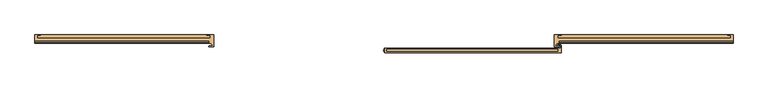
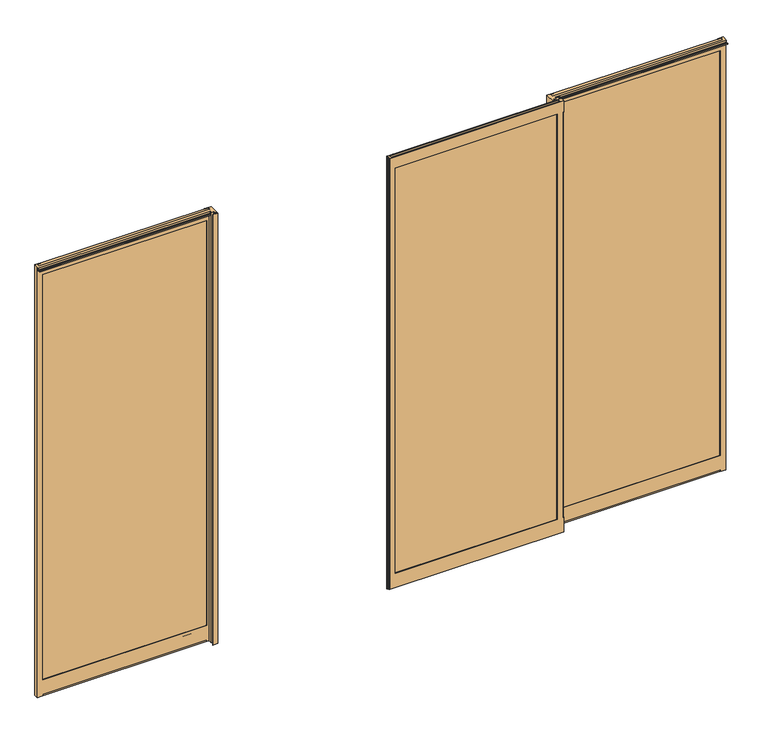
"""IFC4 building model written with IfcOpenShell, lengths in millimetres: door geometry, Otomatik Kapı-Tek Kanat : Otomatik Kapı - Tek Kanat."""

from ifc_helpers import new_model, si_unit, point, frame, frame_2d, origin, place, context, project, spatial, polyline, circle_curve, trimmed, segment, composite_curve, outline, extrude, source, transform, mapped, element, save
from ifc_brep_helpers import plane_surface, cylinder_surface, revolved_surface, advanced_brep


def door_bd07e04d(model_context):
    return source(origin(), model_context, "Body", "SolidModel", [
        advanced_brep(
        [(1555.0015, -107.5, 0.0), (1580.0, -107.5, 0.0), (1580.0, -127.5, 0.0), (1555.0015331, -127.5, 0.0), (1555.0015331, -125.4999765, 0.0), (801.3014669, -125.4999173, 0.0), (801.3014669, -127.5, 0.0), (791.2999735, -127.5, 0.0), (791.2999735, -145.3999231, 0.0), (781.2999977, -145.3999231, 0.0), (781.2999977, -148.5928431, 0.0), (776.0928913, -153.7999496, 0.0), (773.3, -153.7999496, 0.0), (773.3, -156.8999681, 0.0), (790.3010861, -156.8999681, 0.0), (794.3010782, -159.2093663, 0.0), (794.3010782, -160.4999631, 0.0), (771.3, -160.4999631, 0.0), (771.3, -107.5, 0.0), (801.3015, -107.5, 0.0), (801.3015, -109.5000196, 0.0), (1555.0015, -109.4993325, 0.0), (1555.0015331, -127.4999986, 8.0), (1555.0015331, -125.4999737, 8.0), (1555.0015331, -125.499275, 2045.5000009), (1555.0015331, -125.4999497, 77.9996358), (1555.0015331, -127.4999861, 77.9996641), (1555.0015331, -127.4996356, 2045.5000009), (1570.0015, -109.4992492, 62.9982401), (1570.0015, -125.499955, 62.9982401), (1570.0015, -125.499275, 2060.5013187), (1570.0015, -109.4966078, 2060.5013187), (1570.0015, -109.4993325, 2091.0), (1570.0015, -109.4993325, 2089.5000015), (1570.0015, -120.9996409, 2089.5000015), (1570.0015, -122.4996398, 2091.0003428), (1555.0015, -109.4993325, 8.0), (1555.0015, -107.4999999, 8.0), (1555.0015, -107.5, 2091.0), (1555.0015, -107.4999825, 2089.5000015), (1555.0015, -109.4993325, 2089.5000015), (1555.0015, -109.4993325, 2091.0), (1555.0015, -107.4999825, 2045.500003), (1555.0015, -107.4999993, 77.9999376), (1555.0015, -109.4992286, 77.9999379), (1555.0015, -109.4966078, 2045.500003), (801.3015, -107.4999999, 8.0), (801.3015, -109.5000063, 8.0), (801.3015, -109.5000196, 2091.0), (801.3015, -109.5000196, 2089.5000015), (801.3015, -107.4999825, 2089.5000015), (801.3015, -107.5, 2091.0), (801.3015, -109.4966078, 2045.500003), (801.3015, -109.4998895, 77.9999379), (801.3015, -107.4999993, 77.9999376), (801.3015, -107.4999825, 2045.500003), (786.3, -125.4998977, 62.9982401), (786.3, -109.4999153, 62.9982401), (786.3, -109.4966078, 2060.5013187), (786.3, -125.499275, 2060.5013187), (786.3, -122.4996398, 2091.0003428), (786.3, -120.9996409, 2089.5000015), (786.3, -109.5000196, 2089.5000015), (786.3, -109.5000196, 2091.0), (801.3014669, -125.5003878, 8.0), (801.3014669, -127.4999986, 8.0), (801.3014669, -127.4996356, 2045.5000009), (801.3014669, -127.4999861, 77.9996641), (801.3014669, -125.4998928, 77.9996358), (801.3014669, -125.499275, 2045.5000009), (791.2999735, -127.4996356, 2088.5000006), (791.2999735, -131.9000049, 2088.5000006), (791.2999735, -131.9000049, 2081.0024373), (791.2999735, -135.4001347, 2077.4999998), (791.2999735, -145.0000043, 2077.4999987), (791.2999735, -145.0000043, 2082.9999987), (791.2999735, -143.0000044, 2082.9999987), (791.2999735, -143.0000044, 2079.9999989), (791.2999735, -135.4000924, 2079.9999989), (791.2999735, -134.3999191, 2081.0001307), (791.2999735, -134.3999191, 2091.0003428), (791.2999735, -145.3999231, 2091.0), (781.2999977, -145.3999231, 2091.0), (771.3, -160.4999631, 2091.0), (794.3010782, -160.4999631, 2091.0), (1580.0, -107.5, 2091.0), (1580.0, -134.3999191, 2091.0003428), (1580.0, -134.3999191, 2081.0001307), (1580.0, -135.4000924, 2079.9999572), (1580.0, -143.0000044, 2079.9999989), (1580.0, -143.0000044, 2082.9999987), (1580.0, -145.0000043, 2082.9999987), (1580.0, -145.0000043, 2077.4999987), (1580.0, -135.4001347, 2077.4999987), (1580.0, -131.9000049, 2081.0024373), (1580.0, -131.9000049, 2088.5000006), (1580.0, -127.4996356, 2088.5000006), (771.3, -107.5, 2091.0), (794.3010782, -159.2093663, 2091.0003428), (790.3010861, -156.8999681, 2091.0003428), (773.3, -156.8999681, 2091.0003428), (773.3, -153.7999496, 2091.0003428), (776.0928913, -153.7999496, 2091.0003428), (781.2999977, -148.5928431, 2091.0003428)],
        [
            (0, 1),
            (1, 2),
            (2, 3),
            (3, 4),
            (4, 5),
            (5, 6),
            (6, 7),
            (7, 8),
            (8, 9),
            (9, 10),
            (10, 11),
            (11, 12),
            (12, 13),
            (13, 14),
            (14, 15),
            (15, 16),
            (16, 17),
            (17, 18),
            (18, 19),
            (19, 20),
            (20, 21),
            (21, 0),
            (3, 22),
            (22, 23),
            (23, 4),
            (24, 25),
            (25, 26),
            (26, 27),
            (27, 24),
            (28, 29),
            (29, 30),
            (30, 31),
            (31, 28),
            (32, 33),
            (33, 34),
            (34, 35),
            (35, 32),
            (21, 36),
            (36, 37),
            (37, 0),
            (38, 39),
            (39, 40),
            (40, 41),
            (41, 38),
            (42, 43),
            (43, 44),
            (44, 45),
            (45, 42),
            (19, 46),
            (46, 47),
            (47, 20),
            (48, 49),
            (49, 50),
            (50, 51),
            (51, 48),
            (52, 53),
            (53, 54),
            (54, 55),
            (55, 52),
            (56, 57),
            (57, 58),
            (58, 59),
            (59, 56),
            (60, 61),
            (61, 62),
            (62, 63),
            (63, 60),
            (5, 64),
            (64, 65),
            (65, 6),
            (66, 67),
            (67, 68),
            (68, 69),
            (69, 66),
            (70, 71),
            (71, 72),
            (72, 73, circle_curve(frame((791.2999735, -135.4001351, 2081.0001307), z_axis=(-1.0, 0.0, 0.0), x_axis=(0.0, 0.0, 1.0)), 3.5001309)),
            (73, 74),
            (74, 75),
            (75, 76),
            (76, 77),
            (77, 78),
            (78, 79, circle_curve(frame((791.2999735, -135.4000925, 2081.0001307), z_axis=(1.0, 0.0, 0.0), x_axis=(0.0, 0.0, 1.0)), 1.0001735)),
            (79, 80),
            (80, 81),
            (81, 8),
            (7, 70),
            (82, 9),
            (81, 82),
            (83, 17),
            (16, 84),
            (84, 83),
            (45, 52),
            (55, 42),
            (30, 59),
            (58, 31),
            (27, 66),
            (69, 24),
            (25, 68),
            (67, 26),
            (56, 29),
            (28, 57),
            (43, 54),
            (53, 44),
            (1, 85),
            (85, 86),
            (86, 87),
            (87, 88, circle_curve(frame((1580.0, -135.4000925, 2081.0001307), z_axis=(-1.0, 0.0, 0.0), x_axis=(0.0, 0.0, 1.0)), 1.0001735)),
            (88, 89),
            (89, 90),
            (90, 91),
            (91, 92),
            (92, 93),
            (93, 94, circle_curve(frame((1580.0, -135.4001351, 2081.0001307), z_axis=(1.0, 0.0, 0.0), x_axis=(0.0, 0.0, 1.0)), 3.5001309)),
            (94, 95),
            (95, 96),
            (96, 2),
            (83, 97),
            (97, 18),
            (41, 32),
            (35, 60),
            (63, 48),
            (51, 97),
            (84, 98),
            (98, 99),
            (99, 100),
            (100, 101),
            (101, 102),
            (102, 103),
            (103, 82),
            (80, 86),
            (85, 38),
            (37, 46),
            (50, 39),
            (40, 33),
            (62, 49),
            (96, 70),
            (65, 22),
            (34, 61),
            (95, 71),
            (94, 72),
            (93, 73),
            (92, 74),
            (91, 75),
            (90, 76),
            (89, 77),
            (88, 78),
            (87, 79),
            (103, 10),
            (102, 11),
            (101, 12),
            (100, 13),
            (99, 14),
            (98, 15),
            (36, 47),
            (23, 64),
        ],
        [
            plane_surface(frame((1580.0, -107.5, 0.0), z_axis=(0.0, 0.0, -1.0), x_axis=(0.0, -1.0, 0.0))),
            plane_surface(frame((1555.0015331, -127.5, 2091.0), z_axis=(-1.0, 0.0, 0.0), x_axis=(0.0, 0.0, -1.0))),
            plane_surface(frame((1570.0015, -125.4999765, 2091.0), z_axis=(-1.0, 0.0, 0.0), x_axis=(0.0, 0.0, -1.0))),
            plane_surface(frame((1555.0015, -109.4993325, 2091.0), z_axis=(-1.0, 0.0, 0.0), x_axis=(0.0, 0.0, -1.0))),
            plane_surface(frame((801.3015, -107.5, 2091.0), z_axis=(1.0, 0.0, 0.0), x_axis=(0.0, 0.0, -1.0))),
            plane_surface(frame((786.3, -109.5000196, 2091.0), z_axis=(1.0, 0.0, 0.0), x_axis=(0.0, 0.0, -1.0))),
            plane_surface(frame((801.3014669, -125.4999173, 2091.0), z_axis=(1.0, 0.0, 0.0), x_axis=(0.0, 0.0, -1.0))),
            plane_surface(frame((791.2999735, -127.5, 2091.0), z_axis=(1.0, 0.0, 0.0), x_axis=(0.0, 0.0, -1.0))),
            plane_surface(frame((791.2999735, -145.3999231, 2091.0), z_axis=(0.0, -1.0, 0.0), x_axis=(0.0, 0.0, -1.0))),
            plane_surface(frame((794.3010782, -160.4999631, 2091.0), z_axis=(0.0, -1.0, 0.0), x_axis=(0.0, 0.0, -1.0))),
            plane_surface(frame((1580.0, -107.4999825, 2045.500003), z_axis=(0.0, 0.0, -1.0), x_axis=(-1.0, 0.0, 0.0))),
            plane_surface(frame((1580.0, -109.4966078, 2060.5013187), z_axis=(0.0, 0.0, -1.0), x_axis=(-1.0, 0.0, 0.0))),
            plane_surface(frame((1580.0, -125.499275, 2045.5000009), z_axis=(0.0, 0.0, -1.0), x_axis=(-1.0, 0.0, 0.0))),
            plane_surface(frame((1580.0, -127.5, 77.9996641), z_axis=(0.0, 1.4132729652639372e-05, 0.999999999900133), x_axis=(-1.0, 0.0, 0.0))),
            plane_surface(frame((1580.0, -125.4999765, 62.9982401), z_axis=(0.0, 0.0, 1.0), x_axis=(-1.0, 0.0, 0.0))),
            plane_surface(frame((1580.0, -109.4999015, 77.9999379), z_axis=(0.0, 1.674987849023181e-07, 0.999999999999986), x_axis=(-1.0, 0.0, 0.0))),
            plane_surface(frame((1580.0, -107.5, 2091.0), z_axis=(1.0, 0.0, 0.0), x_axis=(0.0, -1.0, 0.0))),
            plane_surface(frame((771.3, -107.5, 2091.0), z_axis=(-1.0, 0.0, 0.0), x_axis=(0.0, -1.0, 0.0))),
            plane_surface(frame((1580.0, -134.3999191, 2091.0003428), z_axis=(0.0, 0.0, 1.0), x_axis=(-1.0, 0.0, 0.0))),
            plane_surface(frame((1580.0, -107.4999825, 2089.5000015), z_axis=(0.0, 1.0, 0.0), x_axis=(-1.0, 0.0, 0.0))),
            plane_surface(frame((1580.0, -109.4966078, 2045.500003), z_axis=(0.0, -1.0, 0.0), x_axis=(-1.0, 0.0, 0.0))),
            plane_surface(frame((1580.0, -125.499275, 2060.5013187), z_axis=(0.0, 1.0, 0.0), x_axis=(-1.0, 0.0, 0.0))),
            plane_surface(frame((1580.0, -127.4996356, 2045.5000009), z_axis=(0.0, -1.0, 0.0), x_axis=(-1.0, 0.0, 0.0))),
            plane_surface(frame((1580.0, -122.4996398, 2091.0003428), z_axis=(0.0, 0.7071874732725993, 0.7070260798911995), x_axis=(-1.0, 0.0, 0.0))),
            plane_surface(frame((1580.0, -120.9996409, 2089.5000015), z_axis=(0.0, 0.0, 1.0), x_axis=(-1.0, 0.0, 0.0))),
            plane_surface(frame((1580.0, -127.4996356, 2088.5000006), z_axis=(0.0, 0.0, -1.0), x_axis=(-1.0, 0.0, 0.0))),
            plane_surface(frame((1580.0, -131.9000049, 2088.5000006), z_axis=(0.0, 1.0, 0.0), x_axis=(-1.0, 0.0, 0.0))),
            cylinder_surface(frame((1580.0, -135.4001351, 2081.0001307), z_axis=(1.0, 0.0, 0.0), x_axis=(0.0, 0.0, 1.0)), 3.5001309),
            plane_surface(frame((1580.0, -135.4001347, 2077.4999987), z_axis=(0.0, 0.0, -1.0), x_axis=(-1.0, 0.0, 0.0))),
            plane_surface(frame((1580.0, -145.0000043, 2077.4999987), z_axis=(0.0, -1.0, 0.0), x_axis=(-1.0, 0.0, 0.0))),
            plane_surface(frame((1580.0, -145.0000043, 2082.9999987), z_axis=(0.0, 0.0, 1.0), x_axis=(-1.0, 0.0, 0.0))),
            plane_surface(frame((1580.0, -143.0000044, 2082.9999987), z_axis=(0.0, 1.0, 0.0), x_axis=(-1.0, 0.0, 0.0))),
            plane_surface(frame((1580.0, -143.0000044, 2079.9999989), z_axis=(0.0, 0.0, 1.0), x_axis=(-1.0, 0.0, 0.0))),
            revolved_surface(polyline([(791.2999735, -135.4000925, 2082.0003042000003), (1580.0, -135.4000925, 2082.0003042000003)]), (1580.0, -135.4000925, 2081.0001307), (-1.0, 0.0, 0.0)),
            plane_surface(frame((1580.0, -134.3999191, 2081.0001307), z_axis=(0.0, -1.0, 0.0), x_axis=(-1.0, 0.0, 0.0))),
            plane_surface(frame((781.2999977, -145.3999231, 2091.0), z_axis=(1.0, 0.0, 0.0), x_axis=(0.0, 0.0, -1.0))),
            plane_surface(frame((781.2999977, -148.5928431, 2091.0), z_axis=(0.7071067811865539, -0.7071067811865412, 0.0), x_axis=(0.0, 0.0, -1.0))),
            plane_surface(frame((776.0928913, -153.7999496, 2091.0), z_axis=(0.0, -1.0, 0.0), x_axis=(0.0, 0.0, -1.0))),
            plane_surface(frame((773.3, -153.7999496, 2091.0), z_axis=(1.0, 0.0, 0.0), x_axis=(0.0, 0.0, -1.0))),
            plane_surface(frame((773.3, -156.8999681, 2091.0), z_axis=(0.0, 1.0, 0.0), x_axis=(0.0, 0.0, -1.0))),
            plane_surface(frame((790.3010861, -156.8999681, 2091.0), z_axis=(0.5000002758229711, 0.8660252445379135, 0.0), x_axis=(0.0, 0.0, -1.0))),
            plane_surface(frame((794.3010782, -159.2093663, 2091.0), z_axis=(1.0, 0.0, 0.0), x_axis=(0.0, 0.0, -1.0))),
            plane_surface(frame((1580.0, -107.5000072, 8.0), z_axis=(0.0, 0.0, -1.0), x_axis=(-1.0, 0.0, 0.0))),
            plane_surface(frame((1580.0, -109.4993325, 8.0), z_axis=(0.0, 1.0, 0.0), x_axis=(-1.0, 0.0, 0.0))),
            plane_surface(frame((1580.0, -125.5003878, 0.0), z_axis=(0.0, -1.0, 0.0), x_axis=(-1.0, 0.0, 0.0))),
            plane_surface(frame((1580.0, -125.5003878, 8.0), z_axis=(0.0, 0.0, -1.0), x_axis=(-1.0, 0.0, 0.0))),
        ],
        [
            (0, [[1, 2, 3, 4, 5, 6, 7, 8, 9, 10, 11, 12, 13, 14, 15, 16, 17, 18, 19, 20, 21, 22]]),
            (1, [[23, 24, 25, -4]]),
            (1, [[26, 27, 28, 29]]),
            (2, [[30, 31, 32, 33]]),
            (2, [[34, 35, 36, 37]]),
            (3, [[38, 39, 40, -22]]),
            (3, [[41, 42, 43, 44]]),
            (3, [[45, 46, 47, 48]]),
            (4, [[49, 50, 51, -20]]),
            (4, [[52, 53, 54, 55]]),
            (4, [[56, 57, 58, 59]]),
            (5, [[60, 61, 62, 63]]),
            (5, [[64, 65, 66, 67]]),
            (6, [[68, 69, 70, -6]]),
            (6, [[71, 72, 73, 74]]),
            (7, [[75, 76, 77, 78, 79, 80, 81, 82, 83, 84, 85, 86, -8, 87]]),
            (8, [[88, -9, -86, 89]]),
            (9, [[90, -17, 91, 92]]),
            (10, [[93, -59, 94, -48]]),
            (11, [[95, -62, 96, -32]]),
            (12, [[97, -74, 98, -29]]),
            (13, [[-27, 99, -72, 100]]),
            (14, [[-60, 101, -30, 102]]),
            (15, [[-46, 103, -57, 104]]),
            (16, [[105, 106, 107, 108, 109, 110, 111, 112, 113, 114, 115, 116, 117, -2]]),
            (17, [[118, 119, -18, -90]]),
            (18, [[-44, 120, -37, 121, -67, 122, -55, 123, -118, -92, 124, 125, 126, 127, 128, 129, 130, -89, -85, 131, -106, 132]]),
            (19, [[-105, -1, -40, 133, -49, -19, -119, -123, -54, 134, -41, -132], [-94, -58, -103, -45]]),
            (20, [[-43, 135, -34, -120]]),
            (20, [[-66, 136, -52, -122]]),
            (20, [[-61, -102, -33, -96], [-47, -104, -56, -93]]),
            (21, [[-31, -101, -63, -95], [-73, -99, -26, -98]]),
            (22, [[-117, 137, -87, -7, -70, 138, -23, -3], [-97, -28, -100, -71]]),
            (23, [[139, -64, -121, -36]]),
            (24, [[-135, -42, -134, -53, -136, -65, -139, -35]]),
            (25, [[140, -75, -137, -116]]),
            (26, [[141, -76, -140, -115]]),
            (27, [[142, -77, -141, -114]]),
            (28, [[143, -78, -142, -113]]),
            (29, [[144, -79, -143, -112]]),
            (30, [[145, -80, -144, -111]]),
            (31, [[146, -81, -145, -110]]),
            (32, [[147, -82, -146, -109]]),
            (33, [[148, -83, -147, -108]]),
            (34, [[-131, -84, -148, -107]]),
            (35, [[149, -10, -88, -130]]),
            (36, [[150, -11, -149, -129]]),
            (37, [[151, -12, -150, -128]]),
            (38, [[152, -13, -151, -127]]),
            (39, [[153, -14, -152, -126]]),
            (40, [[154, -15, -153, -125]]),
            (41, [[-91, -16, -154, -124]]),
            (42, [[-50, -133, -39, 155]]),
            (43, [[-51, -155, -38, -21]]),
            (44, [[-25, 156, -68, -5]]),
            (45, [[-69, -156, -24, -138]]),
        ],
    ),
        extrude(outline(polyline([(788.792088, -114.5000025), (1567.9612743, -114.5000025), (1567.9612743, -124.5000025), (788.792088, -124.5000025), (788.792088, -114.5000025)])), frame((0.0, 0.0, 70.0), z_axis=(0.0, 0.0, 1.0), x_axis=(1.0, 0.0, 0.0)), (0.0, 0.0, 1.0), 1989.0),
        advanced_brep(
        [(-1555.0015, -107.5, 0.0), (-1555.0015, -109.4993325, 0.0), (-801.3015, -109.4966078, 0.0), (-801.3015, -107.5, 0.0), (-771.3, -107.5, 0.0), (-771.3, -160.4999631, 0.0), (-794.3010782, -160.4999631, 0.0), (-794.3010782, -159.2093663, 0.0), (-790.3010861, -156.8999681, 0.0), (-773.3, -156.8999681, 0.0), (-773.3, -153.7999496, 0.0), (-776.0928913, -153.7999496, 0.0), (-781.2999977, -148.5928431, 0.0), (-781.2999977, -145.3999231, 0.0), (-791.2999735, -145.3999231, 0.0), (-791.2999735, -127.5, 0.0), (-801.3014669, -127.5, 0.0), (-801.3014669, -125.4999173, 0.0), (-1555.0015331, -125.499275, 0.0), (-1555.0015331, -127.5, 0.0), (-1580.0, -127.5, 0.0), (-1580.0, -107.5, 0.0), (-1555.0015331, -125.5003878, 8.0), (-1555.0015331, -127.4999986, 8.0), (-1555.0015331, -125.499275, 2045.5000009), (-1555.0015331, -127.4996356, 2045.5000009), (-1555.0015331, -127.4999861, 77.9996641), (-1555.0015331, -125.4999497, 77.9996358), (-1570.0015, -109.4993325, 2091.0), (-1570.0015, -122.4996398, 2091.0003428), (-1570.0015, -120.9996409, 2089.5000015), (-1570.0015, -109.4993325, 2089.5000015), (-1570.0015, -109.4992492, 62.9982401), (-1570.0015, -109.4966078, 2060.5013187), (-1570.0015, -125.499275, 2060.5013187), (-1570.0015, -125.499955, 62.9982401), (-1555.0015, -107.4999999, 8.0), (-1555.0015, -109.4993218, 8.0), (-1555.0015, -107.4999825, 2045.500003), (-1555.0015, -109.4966078, 2045.500003), (-1555.0015, -109.4992286, 77.9999379), (-1555.0015, -107.4999993, 77.9999376), (-1555.0015, -107.5, 2091.0), (-1555.0015, -109.4993325, 2091.0), (-1555.0015, -109.4993325, 2089.5000015), (-1555.0015, -107.4999825, 2089.5000015), (-801.3015, -109.4993325, 8.0), (-801.3015, -107.4999999, 8.0), (-801.3015, -109.4966078, 2045.500003), (-801.3015, -107.4999825, 2045.500003), (-801.3015, -107.4999993, 77.9999376), (-801.3015, -109.4998895, 77.9999379), (-801.3015, -109.5000196, 2091.0), (-801.3015, -107.5, 2091.0), (-801.3015, -107.4999825, 2089.5000015), (-801.3015, -109.5000196, 2089.5000015), (-786.3, -122.4996398, 2091.0003428), (-786.3, -109.5000196, 2091.0), (-786.3, -109.5000196, 2089.5000015), (-786.3, -120.9996409, 2089.5000015), (-786.3, -125.4998977, 62.9982401), (-786.3, -125.499275, 2060.5013187), (-786.3, -109.4966078, 2060.5013187), (-786.3, -109.4999153, 62.9982401), (-801.3014669, -127.4999986, 8.0), (-801.3014669, -125.4999148, 8.0), (-801.3014669, -127.4996356, 2045.5000009), (-801.3014669, -125.499275, 2045.5000009), (-801.3014669, -125.4998928, 77.9996358), (-801.3014669, -127.4999861, 77.9996641), (-791.2999735, -127.4996356, 2088.5000006), (-791.2999735, -145.3999231, 2091.0), (-791.2999735, -134.3999191, 2091.0003428), (-791.2999735, -134.3999191, 2081.0001307), (-791.2999735, -135.4000924, 2079.9999572), (-791.2999735, -143.0000043, 2079.9999989), (-791.2999735, -143.0000043, 2082.9999987), (-791.2999735, -145.0000043, 2082.9999987), (-791.2999735, -145.0000043, 2077.4999987), (-791.2999735, -135.4001347, 2077.4999987), (-791.2999735, -131.9000049, 2081.0024373), (-791.2999735, -131.9000049, 2088.5000006), (-781.2999977, -145.3999231, 2091.0), (-771.3, -160.4999631, 2091.0), (-794.3010782, -160.4999631, 2091.0), (-1580.0, -127.4996356, 2088.5000006), (-1580.0, -131.9000049, 2088.5000006), (-1580.0, -131.9000049, 2081.0024373), (-1580.0, -135.4001347, 2077.4999998), (-1580.0, -145.0000043, 2077.4999987), (-1580.0, -145.0000043, 2082.9999987), (-1580.0, -143.0000043, 2082.9999987), (-1580.0, -143.0000043, 2079.9999989), (-1580.0, -135.400135, 2079.9999989), (-1580.0, -134.3999191, 2081.0001307), (-1580.0, -134.3999191, 2091.0003428), (-1580.0, -107.5, 2091.0), (-771.3, -107.5, 2091.0), (-781.2999977, -148.5928431, 2091.0003428), (-776.0928913, -153.7999496, 2091.0003428), (-773.3, -153.7999496, 2091.0003428), (-773.3, -156.8999681, 2091.0003428), (-790.3010861, -156.8999681, 2091.0003428), (-794.3010782, -159.2093663, 2091.0003428)],
        [
            (0, 1),
            (1, 2),
            (2, 3),
            (3, 4),
            (4, 5),
            (5, 6),
            (6, 7),
            (7, 8),
            (8, 9),
            (9, 10),
            (10, 11),
            (11, 12),
            (12, 13),
            (13, 14),
            (14, 15),
            (15, 16),
            (16, 17),
            (17, 18),
            (18, 19),
            (19, 20),
            (20, 21),
            (21, 0),
            (18, 22),
            (22, 23),
            (23, 19),
            (24, 25),
            (25, 26),
            (26, 27),
            (27, 24),
            (28, 29),
            (29, 30),
            (30, 31),
            (31, 28),
            (32, 33),
            (33, 34),
            (34, 35),
            (35, 32),
            (0, 36),
            (36, 37),
            (37, 1),
            (38, 39),
            (39, 40),
            (40, 41),
            (41, 38),
            (42, 43),
            (43, 44),
            (44, 45),
            (45, 42),
            (2, 46),
            (46, 47),
            (47, 3),
            (48, 49),
            (49, 50),
            (50, 51),
            (51, 48),
            (52, 53),
            (53, 54),
            (54, 55),
            (55, 52),
            (56, 57),
            (57, 58),
            (58, 59),
            (59, 56),
            (60, 61),
            (61, 62),
            (62, 63),
            (63, 60),
            (16, 64),
            (64, 65),
            (65, 17),
            (66, 67),
            (67, 68),
            (68, 69),
            (69, 66),
            (70, 15),
            (14, 71),
            (71, 72),
            (72, 73),
            (73, 74, circle_curve(frame((-791.2999735, -135.4000925, 2081.0001307), z_axis=(-1.0, 0.0, 0.0), x_axis=(0.0, 0.0, 1.0)), 1.0001735)),
            (74, 75),
            (75, 76),
            (76, 77),
            (77, 78),
            (78, 79),
            (79, 80, circle_curve(frame((-791.2999735, -135.4001351, 2081.0001307), z_axis=(1.0, 0.0, 0.0), x_axis=(0.0, 0.0, 1.0)), 3.5001309)),
            (80, 81),
            (81, 70),
            (82, 71),
            (13, 82),
            (83, 84),
            (84, 6),
            (5, 83),
            (38, 49),
            (48, 39),
            (33, 62),
            (61, 34),
            (24, 67),
            (66, 25),
            (26, 69),
            (68, 27),
            (63, 32),
            (35, 60),
            (40, 51),
            (50, 41),
            (20, 85),
            (85, 86),
            (86, 87),
            (87, 88, circle_curve(frame((-1580.0, -135.4001351, 2081.0001307), z_axis=(-1.0, 0.0, 0.0), x_axis=(0.0, 0.0, 1.0)), 3.5001309)),
            (88, 89),
            (89, 90),
            (90, 91),
            (91, 92),
            (92, 93),
            (93, 94, circle_curve(frame((-1580.0, -135.4000925, 2081.0001307), z_axis=(1.0, 0.0, 0.0), x_axis=(0.0, 0.0, 1.0)), 1.0001735)),
            (94, 95),
            (95, 96),
            (96, 21),
            (4, 97),
            (97, 83),
            (42, 96),
            (95, 72),
            (82, 98),
            (98, 99),
            (99, 100),
            (100, 101),
            (101, 102),
            (102, 103),
            (103, 84),
            (97, 53),
            (52, 57),
            (56, 29),
            (28, 43),
            (45, 54),
            (47, 36),
            (55, 58),
            (31, 44),
            (23, 64),
            (70, 85),
            (59, 30),
            (81, 86),
            (80, 87),
            (79, 88),
            (78, 89),
            (77, 90),
            (76, 91),
            (75, 92),
            (74, 93),
            (73, 94),
            (12, 98),
            (11, 99),
            (10, 100),
            (9, 101),
            (8, 102),
            (7, 103),
            (46, 37),
            (65, 22),
        ],
        [
            plane_surface(frame((-1580.0, -107.5, 0.0), z_axis=(0.0, 0.0, -1.0), x_axis=(0.0, -1.0, 0.0))),
            plane_surface(frame((-1555.0015331, -127.5, 2091.0), z_axis=(1.0, 0.0, 0.0), x_axis=(0.0, 0.0, -1.0))),
            plane_surface(frame((-1570.0015, -125.4999765, 2091.0), z_axis=(1.0, 0.0, 0.0), x_axis=(0.0, 0.0, -1.0))),
            plane_surface(frame((-1555.0015, -109.4993325, 2091.0), z_axis=(1.0, 0.0, 0.0), x_axis=(0.0, 0.0, -1.0))),
            plane_surface(frame((-801.3015, -107.5, 2091.0), z_axis=(-1.0, 0.0, 0.0), x_axis=(0.0, 0.0, -1.0))),
            plane_surface(frame((-786.3, -109.5000196, 2091.0), z_axis=(-1.0, 0.0, 0.0), x_axis=(0.0, 0.0, -1.0))),
            plane_surface(frame((-801.3014669, -125.4999173, 2091.0), z_axis=(-1.0, 0.0, 0.0), x_axis=(0.0, 0.0, -1.0))),
            plane_surface(frame((-791.2999735, -127.5, 2091.0), z_axis=(-1.0, 0.0, 0.0), x_axis=(0.0, 0.0, -1.0))),
            plane_surface(frame((-791.2999735, -145.3999231, 2091.0), z_axis=(0.0, -1.0, 0.0), x_axis=(0.0, 0.0, -1.0))),
            plane_surface(frame((-794.3010782, -160.4999631, 2091.0), z_axis=(0.0, -1.0, 0.0), x_axis=(0.0, 0.0, -1.0))),
            plane_surface(frame((-1580.0, -107.4999825, 2045.500003), z_axis=(0.0, 0.0, -1.0), x_axis=(1.0, 0.0, 0.0))),
            plane_surface(frame((-1580.0, -109.4966078, 2060.5013187), z_axis=(0.0, 0.0, -1.0), x_axis=(1.0, 0.0, 0.0))),
            plane_surface(frame((-1580.0, -125.499275, 2045.5000009), z_axis=(0.0, 0.0, -1.0), x_axis=(1.0, 0.0, 0.0))),
            plane_surface(frame((-1580.0, -127.5, 77.9996641), z_axis=(0.0, 1.4132729652639372e-05, 0.999999999900133), x_axis=(1.0, 0.0, 0.0))),
            plane_surface(frame((-1580.0, -125.4999765, 62.9982401), z_axis=(0.0, 0.0, 1.0), x_axis=(1.0, 0.0, 0.0))),
            plane_surface(frame((-1580.0, -109.4999015, 77.9999379), z_axis=(0.0, 1.674987849023181e-07, 0.999999999999986), x_axis=(1.0, 0.0, 0.0))),
            plane_surface(frame((-1580.0, -107.5, 2091.0), z_axis=(-1.0, 0.0, 0.0), x_axis=(0.0, -1.0, 0.0))),
            plane_surface(frame((-771.3, -107.5, 2091.0), z_axis=(1.0, 0.0, 0.0), x_axis=(0.0, -1.0, 0.0))),
            plane_surface(frame((-1580.0, -134.3999191, 2091.0003428), z_axis=(0.0, 0.0, 1.0), x_axis=(1.0, 0.0, 0.0))),
            plane_surface(frame((-1580.0, -107.4999825, 2089.5000015), z_axis=(0.0, 1.0, 0.0), x_axis=(1.0, 0.0, 0.0))),
            plane_surface(frame((-1580.0, -109.4966078, 2045.500003), z_axis=(0.0, -1.0, 0.0), x_axis=(1.0, 0.0, 0.0))),
            plane_surface(frame((-1580.0, -125.499275, 2060.5013187), z_axis=(0.0, 1.0, 0.0), x_axis=(1.0, 0.0, 0.0))),
            plane_surface(frame((-1580.0, -127.4996356, 2045.5000009), z_axis=(0.0, -1.0, 0.0), x_axis=(1.0, 0.0, 0.0))),
            plane_surface(frame((-1580.0, -122.4996398, 2091.0003428), z_axis=(0.0, 0.7071874732725993, 0.7070260798911995), x_axis=(1.0, 0.0, 0.0))),
            plane_surface(frame((-1580.0, -120.9996409, 2089.5000015), z_axis=(0.0, 0.0, 1.0), x_axis=(1.0, 0.0, 0.0))),
            plane_surface(frame((-1580.0, -127.4996356, 2088.5000006), z_axis=(0.0, 0.0, -1.0), x_axis=(1.0, 0.0, 0.0))),
            plane_surface(frame((-1580.0, -131.9000049, 2088.5000006), z_axis=(0.0, 1.0, 0.0), x_axis=(1.0, 0.0, 0.0))),
            cylinder_surface(frame((-1580.0, -135.4001351, 2081.0001307), z_axis=(-1.0, 0.0, 0.0), x_axis=(0.0, 0.0, 1.0)), 3.5001309),
            plane_surface(frame((-1580.0, -135.4001347, 2077.4999987), z_axis=(0.0, 0.0, -1.0), x_axis=(1.0, 0.0, 0.0))),
            plane_surface(frame((-1580.0, -145.0000043, 2077.4999987), z_axis=(0.0, -1.0, 0.0), x_axis=(1.0, 0.0, 0.0))),
            plane_surface(frame((-1580.0, -145.0000043, 2082.9999987), z_axis=(0.0, 0.0, 1.0), x_axis=(1.0, 0.0, 0.0))),
            plane_surface(frame((-1580.0, -143.0000043, 2082.9999987), z_axis=(0.0, 1.0, 0.0), x_axis=(1.0, 0.0, 0.0))),
            plane_surface(frame((-1580.0, -143.0000043, 2079.9999989), z_axis=(0.0, 0.0, 1.0), x_axis=(1.0, 0.0, 0.0))),
            revolved_surface(polyline([(-791.2999735, -135.4000925, 2082.0003042000003), (-1580.0, -135.4000925, 2082.0003042000003)]), (-1580.0, -135.4000925, 2081.0001307), (1.0, 0.0, 0.0)),
            plane_surface(frame((-1580.0, -134.3999191, 2081.0001307), z_axis=(0.0, -1.0, 0.0), x_axis=(1.0, 0.0, 0.0))),
            plane_surface(frame((-781.2999977, -145.3999231, 2091.0), z_axis=(-1.0, 0.0, 0.0), x_axis=(0.0, 0.0, -1.0))),
            plane_surface(frame((-781.2999977, -148.5928431, 2091.0), z_axis=(-0.7071067811865539, -0.7071067811865412, 0.0), x_axis=(0.0, 0.0, -1.0))),
            plane_surface(frame((-776.0928913, -153.7999496, 2091.0), z_axis=(0.0, -1.0, 0.0), x_axis=(0.0, 0.0, -1.0))),
            plane_surface(frame((-773.3, -153.7999496, 2091.0), z_axis=(-1.0, 0.0, 0.0), x_axis=(0.0, 0.0, -1.0))),
            plane_surface(frame((-773.3, -156.8999681, 2091.0), z_axis=(0.0, 1.0, 0.0), x_axis=(0.0, 0.0, -1.0))),
            plane_surface(frame((-790.3010861, -156.8999681, 2091.0), z_axis=(-0.5000002758229711, 0.8660252445379135, 0.0), x_axis=(0.0, 0.0, -1.0))),
            plane_surface(frame((-794.3010782, -159.2093663, 2091.0), z_axis=(-1.0, 0.0, 0.0), x_axis=(0.0, 0.0, -1.0))),
            plane_surface(frame((-1580.0, -107.5000072, 8.0), z_axis=(0.0, 0.0, -1.0), x_axis=(1.0, 0.0, 0.0))),
            plane_surface(frame((-1580.0, -109.4993325, 8.0), z_axis=(0.0, 1.0, 0.0), x_axis=(1.0, 0.0, 0.0))),
            plane_surface(frame((-1580.0, -125.5003878, 0.0), z_axis=(0.0, -1.0, 0.0), x_axis=(1.0, 0.0, 0.0))),
            plane_surface(frame((-1580.0, -125.5003878, 8.0), z_axis=(0.0, 0.0, -1.0), x_axis=(1.0, 0.0, 0.0))),
        ],
        [
            (0, [[1, 2, 3, 4, 5, 6, 7, 8, 9, 10, 11, 12, 13, 14, 15, 16, 17, 18, 19, 20, 21, 22]]),
            (1, [[-19, 23, 24, 25]]),
            (1, [[26, 27, 28, 29]]),
            (2, [[30, 31, 32, 33]]),
            (2, [[34, 35, 36, 37]]),
            (3, [[-1, 38, 39, 40]]),
            (3, [[41, 42, 43, 44]]),
            (3, [[45, 46, 47, 48]]),
            (4, [[-3, 49, 50, 51]]),
            (4, [[52, 53, 54, 55]]),
            (4, [[56, 57, 58, 59]]),
            (5, [[60, 61, 62, 63]]),
            (5, [[64, 65, 66, 67]]),
            (6, [[-17, 68, 69, 70]]),
            (6, [[71, 72, 73, 74]]),
            (7, [[75, -15, 76, 77, 78, 79, 80, 81, 82, 83, 84, 85, 86, 87]]),
            (8, [[88, -76, -14, 89]]),
            (9, [[90, 91, -6, 92]]),
            (10, [[-41, 93, -52, 94]]),
            (11, [[-35, 95, -65, 96]]),
            (12, [[-26, 97, -71, 98]]),
            (13, [[99, -73, 100, -28]]),
            (14, [[101, -37, 102, -67]]),
            (15, [[103, -54, 104, -43]]),
            (16, [[-21, 105, 106, 107, 108, 109, 110, 111, 112, 113, 114, 115, 116, 117]]),
            (17, [[-92, -5, 118, 119]]),
            (18, [[120, -116, 121, -77, -88, 122, 123, 124, 125, 126, 127, 128, -90, -119, 129, -56, 130, -60, 131, -30, 132, -45]]),
            (19, [[-120, -48, 133, -57, -129, -118, -4, -51, 134, -38, -22, -117], [-44, -104, -53, -93]]),
            (20, [[-95, -34, -101, -66], [-94, -55, -103, -42]]),
            (20, [[-130, -59, 135, -61]]),
            (20, [[-132, -33, 136, -46]]),
            (21, [[-96, -64, -102, -36], [-97, -29, -100, -72]]),
            (22, [[-20, -25, 137, -68, -16, -75, 138, -105], [-74, -99, -27, -98]]),
            (23, [[-31, -131, -63, 139]]),
            (24, [[-32, -139, -62, -135, -58, -133, -47, -136]]),
            (25, [[-106, -138, -87, 140]]),
            (26, [[-107, -140, -86, 141]]),
            (27, [[-108, -141, -85, 142]]),
            (28, [[-109, -142, -84, 143]]),
            (29, [[-110, -143, -83, 144]]),
            (30, [[-111, -144, -82, 145]]),
            (31, [[-112, -145, -81, 146]]),
            (32, [[-113, -146, -80, 147]]),
            (33, [[-114, -147, -79, 148]]),
            (34, [[-115, -148, -78, -121]]),
            (35, [[-122, -89, -13, 149]]),
            (36, [[-123, -149, -12, 150]]),
            (37, [[-124, -150, -11, 151]]),
            (38, [[-125, -151, -10, 152]]),
            (39, [[-126, -152, -9, 153]]),
            (40, [[-127, -153, -8, 154]]),
            (41, [[-128, -154, -7, -91]]),
            (42, [[155, -39, -134, -50]]),
            (43, [[-2, -40, -155, -49]]),
            (44, [[-18, -70, 156, -23]]),
            (45, [[-137, -24, -156, -69]]),
        ],
    ),
        extrude(outline(polyline([(-788.792088, -114.5000025), (-788.792088, -124.5000025), (-1567.9612743, -124.5000025), (-1567.9612743, -114.5000025), (-788.792088, -114.5000025)])), frame((0.0, 0.0, 70.0), z_axis=(0.0, 0.0, 1.0), x_axis=(1.0, 0.0, 0.0)), (0.0, 0.0, 1.0), 1989.0),
        advanced_brep(
        [(802.5, -155.7669497, 8.0000212), (802.5, -187.3, 8.0000212), (2.5, -187.3, 8.0000212), (2.5, -167.3000082, 8.0000212), (800.5, -167.3, 8.0000212), (800.5, -155.8138546, 8.0000212), (799.4861454, -154.8, 8.0000212), (787.49925, -154.8, 8.0000212), (787.49925, -152.8, 8.0000212), (799.5330503, -152.8, 8.0000212), (787.49925, -180.7974169, 8.0000212), (787.49925, -173.8001834, 8.0000212), (12.4985, -173.8001834, 8.0000212), (12.4985, -180.7974169, 8.0000212), (800.5, -167.3, 2101.0), (2.5, -167.3, 2101.0), (2.5, -187.3, 2101.0), (802.5, -187.3, 2101.0), (802.5, -155.7669497, 2101.0), (799.5330503, -152.8, 2101.0), (787.49925, -152.8, 2101.0), (787.49925, -154.8, 2101.0), (799.4861454, -154.8, 2101.0), (800.5, -155.8138546, 2101.0), (787.49925, -172.299, 2101.0), (787.49925, -182.301, 2101.0), (12.4985, -182.301, 2101.0), (12.4985, -172.299, 2101.0), (802.5, -187.3, 2046.0007973), (802.5, -185.3, 2046.0007973), (802.5, -185.3, 2061.0007973), (802.5, -184.239458, 2061.0007973), (802.5, -184.239458, 62.9982446), (802.5, -185.3, 62.9982446), (802.5, -185.3, 78.000055), (802.5, -187.3, 78.000055), (772.4862373, -167.3, 2046.0004744), (772.4862373, -167.3, 77.9999799), (772.4862373, -169.2993721, 77.9999799), (772.4862373, -169.2993721, 2046.0004744), (787.49925, -169.2993721, 2061.0007973), (12.4985, -169.2993721, 2061.0007973), (12.4985, -169.2993721, 62.9982446), (787.49925, -169.2993721, 62.9982446), (27.4985, -169.2993721, 77.9999799), (27.4985, -169.2993721, 2046.0004744), (787.49925, -185.3, 62.9982446), (787.49925, -185.3, 2061.0007973), (787.49925, -172.299, 2092.5), (787.49925, -182.301, 2092.5), (787.49925, -180.7974169, 33.4998483), (787.49925, -173.8001834, 33.4998483), (802.3103756, -185.3, 2046.0007973), (802.3103756, -185.3, 2061.0007973), (802.3103756, -185.3, 62.9982446), (802.3103756, -185.3, 78.000055), (12.4985, -185.3, 62.9982446), (12.4985, -185.3, 2061.0007973), (772.4985, -185.3, 2046.0007973), (27.4985, -185.3, 2046.0007973), (27.4985, -185.3, 78.000055), (772.4985, -185.3, 78.000055), (772.4985, -187.3, 78.000055), (772.4985, -187.3, 2046.0007973), (799.439458, -187.3, 78.000055), (799.439458, -187.3, 2046.0007973), (27.4985, -187.3, 78.000055), (27.4985, -187.3, 2046.0007973), (27.4985, -167.3, 2046.0004744), (27.4985, -167.3, 77.9999799), (12.4985, -182.301, 2092.5), (12.4985, -172.299, 2092.5), (12.4985, -173.8001834, 33.4998483), (12.4985, -180.7974169, 33.4998483)],
        [
            (0, 1),
            (1, 2),
            (2, 3),
            (3, 4),
            (4, 5),
            (5, 6, circle_curve(frame((799.4861454, -155.8138546, 8.0000212), z_axis=(0.0, 0.0, 1.0), x_axis=(1.0, 0.0, 0.0)), 1.0138546)),
            (6, 7),
            (7, 8),
            (8, 9),
            (9, 0, circle_curve(frame((799.5330503, -155.7669497, 8.0000212), z_axis=(0.0, 0.0, -1.0), x_axis=(1.0, 0.0, 0.0)), 2.9669497)),
            (10, 11),
            (11, 12),
            (12, 13),
            (13, 10),
            (14, 15),
            (15, 16),
            (16, 17),
            (17, 18),
            (18, 19, circle_curve(frame((799.5330503, -155.7669497, 2101.0), z_axis=(0.0, 0.0, 1.0), x_axis=(1.0, 0.0, 0.0)), 2.9669497)),
            (19, 20),
            (20, 21),
            (21, 22),
            (22, 23, circle_curve(frame((799.4861454, -155.8138546, 2101.0), z_axis=(0.0, 0.0, -1.0), x_axis=(1.0, 0.0, 0.0)), 1.0138546)),
            (23, 14),
            (24, 25),
            (25, 26),
            (26, 27),
            (27, 24),
            (17, 28),
            (28, 29),
            (29, 30),
            (30, 31),
            (31, 32),
            (32, 33),
            (33, 34),
            (34, 35),
            (35, 1),
            (0, 18),
            (8, 20),
            (19, 9),
            (7, 21),
            (36, 37),
            (37, 38),
            (38, 39),
            (39, 36),
            (40, 41),
            (41, 42),
            (42, 43),
            (43, 40),
            (38, 44),
            (44, 45),
            (45, 39),
            (43, 46),
            (46, 47),
            (47, 40),
            (24, 48),
            (48, 49),
            (49, 25),
            (10, 50),
            (50, 51),
            (51, 11),
            (29, 52),
            (52, 53),
            (53, 30),
            (33, 54),
            (54, 55),
            (55, 34),
            (46, 56),
            (56, 57),
            (57, 47),
            (58, 59),
            (59, 60),
            (60, 61),
            (61, 58),
            (61, 62),
            (62, 63),
            (63, 58),
            (16, 2),
            (35, 64),
            (64, 65),
            (65, 28),
            (62, 66),
            (66, 67),
            (67, 63),
            (14, 4),
            (3, 15),
            (36, 68),
            (68, 69),
            (69, 37),
            (6, 22),
            (23, 5),
            (52, 65, circle_curve(frame((799.439458, -184.239458, 2046.0007973), z_axis=(0.0, 0.0, -1.0), x_axis=(1.0, 0.0, 0.0)), 3.060542)),
            (64, 55, circle_curve(frame((799.439458, -184.239458, 78.000055), z_axis=(0.0, 0.0, 1.0), x_axis=(1.0, 0.0, 0.0)), 3.060542)),
            (54, 32, circle_curve(frame((799.439458, -184.239458, 62.9982446), z_axis=(0.0, 0.0, 1.0), x_axis=(1.0, 0.0, 0.0)), 3.060542)),
            (31, 53, circle_curve(frame((799.439458, -184.239458, 2061.0007973), z_axis=(0.0, 0.0, -1.0), x_axis=(1.0, 0.0, 0.0)), 3.060542)),
            (49, 70),
            (70, 26),
            (48, 71),
            (71, 70),
            (27, 71),
            (45, 68),
            (57, 41),
            (67, 59),
            (60, 66),
            (42, 56),
            (69, 44),
            (51, 72),
            (72, 12),
            (50, 73),
            (73, 72),
            (13, 73),
        ],
        [
            plane_surface(frame((802.5, -167.3, 8.0000212), z_axis=(0.0, 0.0, -1.0), x_axis=(0.0, -1.0, 0.0))),
            plane_surface(frame((802.5, -167.3, 2101.0), z_axis=(0.0, 0.0, 1.0), x_axis=(0.0, -1.0, 0.0))),
            plane_surface(frame((802.5, -184.239458, 8.0000212), z_axis=(1.0, 0.0, 0.0), x_axis=(0.0, 0.0, 1.0))),
            plane_surface(frame((799.5330503, -152.8, 8.0000212), z_axis=(0.0, 1.0, 0.0), x_axis=(0.0, 0.0, 1.0))),
            plane_surface(frame((787.49925, -152.8, 8.0000212), z_axis=(-1.0, 0.0, 0.0), x_axis=(0.0, 0.0, 1.0))),
            plane_surface(frame((772.4862373, -167.3, 8.0000212), z_axis=(-1.0, 0.0, 0.0), x_axis=(0.0, 0.0, 1.0))),
            plane_surface(frame((772.4862373, -169.2993721, 8.0000212), z_axis=(0.0, -1.0, 0.0), x_axis=(0.0, 0.0, 1.0))),
            plane_surface(frame((787.49925, -169.2993721, 8.0000212), z_axis=(-1.0, 0.0, 0.0), x_axis=(0.0, 0.0, 1.0))),
            plane_surface(frame((787.49925, -185.3, 8.0000212), z_axis=(0.0, 1.0, 0.0), x_axis=(0.0, 0.0, 1.0))),
            plane_surface(frame((772.4985, -185.3, 8.0000212), z_axis=(-1.0, 0.0, 0.0), x_axis=(0.0, 0.0, 1.0))),
            plane_surface(frame((772.4985, -187.3, 8.0000212), z_axis=(0.0, -1.0, 0.0), x_axis=(0.0, 0.0, 1.0))),
            plane_surface(frame((800.5, -167.3, 8.0000212), z_axis=(0.0, 1.0, 0.0), x_axis=(0.0, 0.0, 1.0))),
            plane_surface(frame((787.49925, -154.8, 8.0000212), z_axis=(0.0, -1.0, 0.0), x_axis=(0.0, 0.0, 1.0))),
            plane_surface(frame((800.5, -155.8138546, 8.0000212), z_axis=(-1.0, 0.0, 0.0), x_axis=(0.0, 0.0, 1.0))),
            cylinder_surface(frame((799.439458, -184.239458, 8.0000212), z_axis=(0.0, 0.0, -1.0), x_axis=(1.0, 0.0, 0.0)), 3.060542),
            cylinder_surface(frame((799.5330503, -155.7669497, 8.0000212), z_axis=(0.0, 0.0, -1.0), x_axis=(1.0, 0.0, 0.0)), 2.9669497),
            revolved_surface(polyline([(800.5, -155.8138546, 2101.0), (800.5, -155.8138546, 8.0000212)]), (799.4861454, -155.8138546, 8.0000212), (0.0, 0.0, 1.0)),
            plane_surface(frame((2.5, -167.3, 2101.0), z_axis=(-1.0, 0.0, 0.0), x_axis=(0.0, -1.0, 0.0))),
            plane_surface(frame((802.5, -182.301, 2101.0), z_axis=(0.0, 1.0, 0.0), x_axis=(-1.0, 0.0, 0.0))),
            plane_surface(frame((802.5, -182.301, 2092.5), z_axis=(0.0, 0.0, 1.0), x_axis=(-1.0, 0.0, 0.0))),
            plane_surface(frame((802.5, -172.299, 2092.5), z_axis=(0.0, -1.0, 0.0), x_axis=(-1.0, 0.0, 0.0))),
            plane_surface(frame((802.5, -167.3, 2046.0004744), z_axis=(0.0, 0.0, -1.0), x_axis=(-1.0, 0.0, 0.0))),
            plane_surface(frame((802.5, -169.3, 2061.0007973), z_axis=(0.0, 0.0, -1.0), x_axis=(-1.0, 0.0, 0.0))),
            plane_surface(frame((802.5, -185.3, 2046.0007973), z_axis=(0.0, 0.0, -1.0), x_axis=(-1.0, 0.0, 0.0))),
            plane_surface(frame((802.5, -187.3, 78.000055), z_axis=(0.0, 0.0, 1.0), x_axis=(-1.0, 0.0, 0.0))),
            plane_surface(frame((802.5, -185.3, 62.9982446), z_axis=(0.0, 0.0, 1.0), x_axis=(-1.0, 0.0, 0.0))),
            plane_surface(frame((802.5, -169.3000224, 77.9999799), z_axis=(0.0, 0.0, 1.0), x_axis=(-1.0, 0.0, 0.0))),
            plane_surface(frame((802.5, -173.8001834, 8.0000212), z_axis=(0.0, -1.0, 0.0), x_axis=(-1.0, 0.0, 0.0))),
            plane_surface(frame((802.5, -173.8001834, 33.4998483), z_axis=(0.0, 0.0, -1.0), x_axis=(-1.0, 0.0, 0.0))),
            plane_surface(frame((802.5, -180.7974169, 33.4998483), z_axis=(0.0, 1.0, 0.0), x_axis=(-1.0, 0.0, 0.0))),
            plane_surface(frame((27.4985, -187.3, 8.0000212), z_axis=(1.0, 0.0, 0.0), x_axis=(0.0, 0.0, 1.0))),
            plane_surface(frame((12.4985, -185.3, 8.0000212), z_axis=(1.0, 0.0, 0.0), x_axis=(0.0, 0.0, 1.0))),
            plane_surface(frame((27.4985, -169.3, 8.0000212), z_axis=(1.0, 0.0, 0.0), x_axis=(0.0, 0.0, 1.0))),
        ],
        [
            (0, [[1, 2, 3, 4, 5, 6, 7, 8, 9, 10], [11, 12, 13, 14]]),
            (1, [[15, 16, 17, 18, 19, 20, 21, 22, 23, 24], [25, 26, 27, 28]]),
            (2, [[-18, 29, 30, 31, 32, 33, 34, 35, 36, 37, -1, 38]]),
            (3, [[39, -20, 40, -9]]),
            (4, [[41, -21, -39, -8]]),
            (5, [[42, 43, 44, 45]]),
            (6, [[46, 47, 48, 49], [50, 51, 52, -44]]),
            (7, [[-49, 53, 54, 55]]),
            (7, [[56, 57, 58, -25]]),
            (7, [[59, 60, 61, -11]]),
            (8, [[62, 63, 64, -31]]),
            (8, [[65, 66, 67, -35]]),
            (8, [[68, 69, 70, -54], [71, 72, 73, 74]]),
            (9, [[-74, 75, 76, 77]]),
            (10, [[78, -2, -37, 79, 80, 81, -29, -17], [-76, 82, 83, 84]]),
            (11, [[85, -4, 86, -15], [-42, 87, 88, 89]]),
            (12, [[90, -22, -41, -7]]),
            (13, [[-85, -24, 91, -5]]),
            (14, [[-63, 92, -80, 93, -66, 94, -33, 95]]),
            (15, [[-40, -19, -38, -10]]),
            (16, [[-91, -23, -90, -6]]),
            (17, [[-16, -86, -3, -78]]),
            (18, [[96, 97, -26, -58]]),
            (19, [[98, 99, -96, -57]]),
            (20, [[-28, 100, -98, -56]]),
            (21, [[-52, 101, -87, -45]]),
            (22, [[-64, -95, -32]]),
            (22, [[102, -46, -55, -70]]),
            (23, [[-84, 103, -71, -77]]),
            (23, [[-81, -92, -62, -30]]),
            (24, [[-67, -93, -79, -36]]),
            (24, [[-73, 104, -82, -75]]),
            (25, [[-94, -65, -34]]),
            (25, [[105, -68, -53, -48]]),
            (26, [[-89, 106, -50, -43]]),
            (27, [[107, 108, -12, -61]]),
            (28, [[109, 110, -107, -60]]),
            (29, [[-14, 111, -109, -59]]),
            (30, [[-103, -83, -104, -72]]),
            (31, [[-97, -99, -100, -27]]),
            (31, [[-105, -47, -102, -69]]),
            (31, [[-108, -110, -111, -13]]),
            (32, [[-101, -51, -106, -88]]),
        ],
    ),
        extrude(outline(polyline([(14.9985, -170.3000147), (784.0, -170.3000147), (784.0, -180.2993696), (14.9985, -180.2993696), (14.9985, -170.3000147)])), frame((0.0, 0.0, 65.4907153), z_axis=(0.0, 0.0, 1.0), x_axis=(1.0, 0.0, 0.0)), (0.0, 0.0, 1.0), 1993.010082),
        extrude(outline(polyline([(-170.3000393, 2058.9584681), (-170.3000367, 2075.4578872), (-169.3000368, 2075.4578872), (-169.3000392, 2060.1996761), (-167.7000392, 2060.1994116), (-167.7000392, 2059.1856312), (-170.3000393, 2058.9584681)])), frame((2.5, 0.0, 0.0), z_axis=(1.0, 0.0, 0.0), x_axis=(0.0, 1.0, 0.0)), (0.0, 0.0, 1.0), 800.0),
        extrude(outline(polyline([(-170.3000147, 79.2411881), (-167.7000146, 79.0140251), (-167.7000146, 78.0002446), (-169.3000145, 77.9999802), (-169.3000145, 62.7412326), (-170.3000121, 62.7417691), (-170.3000147, 79.2411881)])), frame((2.5, 0.0, 0.0), z_axis=(1.0, 0.0, 0.0), x_axis=(0.0, 1.0, 0.0)), (0.0, 0.0, 1.0), 800.0),
        extrude(outline(polyline([(28.9063127, -170.5002199), (16.8469137, -170.5002199), (16.8469137, -169.3), (27.4985, -169.3), (27.4985, -167.6994998), (28.6110353, -167.6994998), (28.9063127, -170.5002199)])), frame((0.0, 0.0, 8.0000212), z_axis=(0.0, 0.0, 1.0), x_axis=(1.0, 0.0, 0.0)), (0.0, 0.0, 1.0), 2092.9999788),
        extrude(outline(composite_curve([segment(polyline([(2.5, -186.2971769), (0.5, -186.2971769), (0.5, -182.1216576)]), True, "CONTINUOUS"), segment(trimmed(circle_curve(frame_2d((-2.5, -182.1216576)), 3.0), [point((0.5, -182.1216576))], [point((-1.0, -179.5235814))], True, "CARTESIAN"), True, "CONTINUOUS"), segment(polyline([(-1.0, -179.5235814), (-3.5821899, -178.0327534)]), True, "CONTINUOUS"), segment(trimmed(circle_curve(frame_2d((-3.1542447, -177.2915306)), 0.8558903), [point((-3.5821899, -178.0327534))], [point((-3.5821899, -176.5503078))], False, "CARTESIAN"), True, "CONTINUOUS"), segment(polyline([(-3.5821899, -176.5503078), (-1.0, -175.0594798)]), True, "CONTINUOUS"), segment(trimmed(circle_curve(frame_2d((-2.5, -172.4614036)), 3.0), [point((-1.0, -175.0594798))], [point((0.5, -172.4614036))], True, "CARTESIAN"), True, "CONTINUOUS"), segment(polyline([(0.5, -172.4614036), (0.5, -168.2971769), (2.5, -168.2971769), (2.5, -186.2971769)]), True, "CONTINUOUS")], self_intersect=False)), frame((0.0, 0.0, 8.0000212), z_axis=(0.0, 0.0, 1.0), x_axis=(1.0, 0.0, 0.0)), (0.0, 0.0, 1.0), 2092.9999788),
        extrude(outline(polyline([(783.1860852, -169.2999998), (783.1860852, -170.50022), (771.0906874, -170.50022), (771.385912, -167.6999998), (772.5, -167.6999998), (772.5, -169.2999998), (783.1860852, -169.2999998)])), frame((0.0, 0.0, 8.0000212), z_axis=(0.0, 0.0, 1.0), x_axis=(1.0, 0.0, 0.0)), (0.0, 0.0, 1.0), 2092.9999788),
    ])


if __name__ == "__main__":
    model = new_model("IFC4")
    model_context = context("Model", 3, world=origin())
    ifc_project = project(units=[si_unit("LENGTHUNIT", "METRE", prefix="MILLI")], contexts=[model_context])
    site = spatial("IfcSite", under=ifc_project)
    building = spatial("IfcBuilding", under=site)
    placement = place(None, origin())
    door_shape = door_bd07e04d(model_context)
    element("IfcDoor", 1, ObjectType="Otomatik Kapı-Tek Kanat : Otomatik Kapı - Tek Kanat", at=placement, inside=building, context=model_context, shape_type="MappedRepresentation", body=[
        mapped(door_shape, transform((0.0, 0.0, 0.0), x_axis=(1.0, 0.0, 0.0), y_axis=(0.0, 1.0, 0.0), z_axis=(0.0, 0.0, 1.0))),
    ])
    save(model, "model.ifc")

# Revit data of these elements
# Type "Otomatik Kapı-Tek Kanat : Otomatik Kapı - Tek Kanat"
#   Type Mark = "41"
#   Uniformat II Description = "Exterior Doors"
#   Uniformat II Code = "B2030"
#   Uniclass 2015 Name = "Sliding doorset systems"
#   Uniclass 2015 Code = "Ss_25_30_20_77"
#   Uniclass 2.0 Description = "Sliding Doorset Systems"
#   Uniclass 2.0 Code = "SS-25-30-20-77"
#   Uniclass 1.4 Description = "Doors"
#   Uniclass 1.4 Code = "L411"
#   UNSPSC Code = "30171510"
#   Technical description = "https://media.gilgendoorsystems.com/download/NcPWaystFgYr"
#   QR code = "https://bimobject.com/gilgen/product/sliding_door_psa_bi-parting_withsidepanels_onwall"
#   Product url = "https://www.gilgendoorsystems.com/en/products-and-systems/automatic-door-systems/sliding-doors/sliding-door-design-slim-frame"
#   Product name = "Automatic Sliding Door (slim frame) - Bi-parting - With side panels - On wall - SL/PSA"
#   Product group = "Automatic Sliding Doors"
#   Product family = "Automatic Sliding Doors"
#   Product data url = "https://bimobject.com/gilgen/product/sliding_door_psa_bi-parting_withsidepanels_onwall"
#   Product certification = "https://www.gilgendoorsystems.com/en/download-centre/tuev-certificates"
#   Product SKU = "Sliding_Door_PSA_Bi-parting_WithSidePanels_Onwall"
#   Product Guid = "e85bef2e-33fe-4a9e-86a7-7fe4a60005b2"
#   OmniClass Description = "Doors"
#   OmniClass Code = "23-17 11 00"
#   Note = "230V/13A Connector socket needed, the operator also needs a voltage-free contacts for opening commande or switching between program functions"
#   NBS Reference Description = "Sliding Doorset Systems"
#   NBS Reference Code = "25-30-20-77"
#   Model = "SL PSA"
#   Material secondary = "Glass"
#   Material main = "Aluminium"
#   Masterformat 2014 Description = "Sliding Aluminum-Framed Glass Doors"
#   Masterformat 2014 Code = "08 32 13"
#   Manufacturer name = "Gilgen"
#   Manufacturer country = "Switzerland"
#   Manufacturer = "Gilgen"
#   Keynote = "08000"
#   Installation instructions = "https://media.gilgendoorsystems.com/product/sl#"
#   IFC Classification = "Door"
#   Design country = "Switzerland"
#   Date of publishing = "08.01.2020 00:00:00"
#   Colours Note = "All colours are available"
#   Bottom Rail Note 2 [instance default] = "For the Drained continuous guide rail There must be flexible tubes on site to take out water (Slope < 1.5 %). The flexible tube connection is thread ½, and a EPDM foil or liquid synthetic material outside and a Air- and vapor-tight foil inside (on site)"
#   Bottom Rail Note [instance default] = "For drained and heated rails a cable from the header to the bottom rail in a M25 pipe is needed"
#   BIMobject category = "Sliding"
#   Assembly Code = "B2030100"
#   Analytic Construction = "<None>"
#   Standard Profile [instance default] = 5.00 cm
#   Rough Width = 313.00 cm
#   Rough Height = 220.00 cm
#   Pocket screen right = 84.07 cm
#   Pocket screen left = 84.07 cm
#   Pocket screen height [instance default] = 208.50 cm
#   Opening distance [instance default] = 0.50 cm
#   Opening Width LB = 160.00 cm
#   Opening Width Control = 160.00 cm
#   Opening Height LH = 220.00 cm
#   Moving leaf right = 80.00 cm
#   Moving leaf left = 80.00 cm
#   Moving leaf height [instance default] = 210.10 cm
#   Inset [instance default] = 0.00 cm
#   Header width = 320.00 cm
#   Header offset right CR = 0.00 cm
#   Header offset left CL = 0.00 cm
#   Header height [instance default] = 14.00 cm
#   Header Right Control = 0.00 cm
#   Header Left Control = 0.00 cm
#   Gap above header control [instance default] = 0.00 cm
#   Gap above header OH = 0.00 cm
#   Height = 220.00 cm
#   Width = 320.00 cm
#   Fixed leaf right = 80.87 cm
#   Fixed leaf left = 80.87 cm
#   Fixed leaf height [instance default] = 209.10 cm
#   CR max = 280.00 cm
#   CL max = 280.00 cm
#   Standard [instance default] = yes
#   Sideplate [instance default] = no
#   Sidecap [instance default] = no
#   Rail 4 [instance default] = no
#   Rail 3 [instance default] = no
#   Rail 2 [instance default] = no
#   Rail 1 [instance default] = no
#   Pocket screen [instance default] = yes
#   Open [instance default] = no
#   Heated [instance default] = no
#   Fixed point [instance default] = yes
#   Edition number = 1
#   Dimension Overconstraint = no
#   Connector [instance default] = no
#   Closing Profile [instance default] = no
#   Mounting Option [instance default] = element 414793
#   Mounting G = element 414798
#   Mounting F = element 414797
#   Mounting E = element 414796
#   Mounting D = element 414795
#   Mounting C = element 414794
#   Mounting B = element 414793
#   Mounting A = element 414792
#   Header Option [instance default] = element 414791
#   Header 2 = element 414791
#   Header 1 = element 414790
#   Guide 5 = element 414803
#   Guide 4 = element 414802
#   Guide 3 = element 414801
#   Guide 2 = element 414800
#   Guide 1 = element 414799
#   Frame material = Finish_Gilgen_Aluminium
#   Bottom Rail Guide [instance default] = element 414799
#   Function = (empty or 0)
#   Wall Closure = (empty or 0)
# Element 1 (IfcDoor, "Otomatik Kapı-Tek Kanat : Otomatik Kapı - Tek Kanat")
#   Materials on its faces: "Finish_Gilgen_Aluminium", "Glass", "Rubber, Natural"
# Materials
#   "Finish_Gilgen_Aluminium": class "Metal", colour RGB 120 120 120, transparency 0, Description = "Aluminium", Cost = 0
#   "Glass": class "Glass", colour RGB 0 128 192, transparency 0.9, Description = "Soda Lime Glass", Cost = 0
#   "Rubber, Natural": class "Plastic", colour RGB 120 120 120, transparency 0, Description = "Natural rubber", Cost = 0
